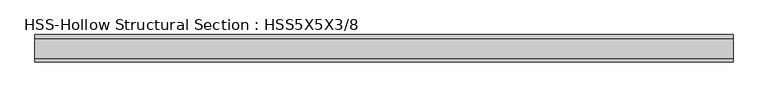
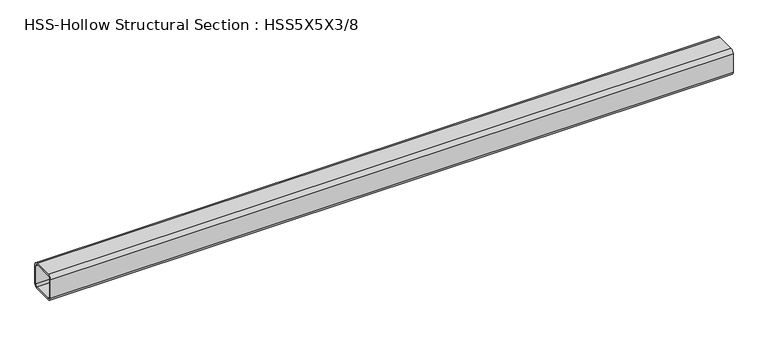
"""IFC4 building model written with IfcOpenShell, lengths in millimetres: member geometry, HSS-Hollow Structural Section : HSS5X5X3/8."""

import ifcopenshell
import ifcopenshell.guid

model = None  # the IFC model being written
_history = None  # IfcOwnerHistory: only IFC2X3 demands one
_inside = {}  # id of a spatial element -> (the spatial element, [elements in it])
_under = {}  # id of a project, library or spatial element -> (it, [spatial elements below it])
_declared = {}  # id of a project -> (the project, [libraries it declares])
_typed = {}  # id of a type object -> (the type object, [elements of that type])
_made_of = {}  # id of a material, layer set ... -> (it, [elements and type objects made of it])


def new_model(schema):
    """Start an empty IFC model of exactly this schema.

    Asked for "IFC4X3", IfcOpenShell would pick the latest addendum, in which some entities
    have other attributes; the version numbers below select the first issue.
    IFC2X3 requires an IfcOwnerHistory on every rooted entity: one is made here for all.
    """
    global model, _history
    if schema == "IFC4X3":
        model = ifcopenshell.file(schema_version=(4, 3, 0, 0))
    else:
        model = ifcopenshell.file(schema=schema)
    _inside.clear()
    _under.clear()
    _declared.clear()
    _typed.clear()
    _made_of.clear()
    _history = None
    if model.schema == "IFC2X3":
        org = make("IfcOrganization", Name="unknown")
        user = make(
            "IfcPersonAndOrganization",
            ThePerson=make("IfcPerson", FamilyName="unknown"),
            TheOrganization=org,
        )
        app = make(
            "IfcApplication",
            ApplicationDeveloper=org,
            Version="unknown",
            ApplicationFullName="unknown",
            ApplicationIdentifier="unknown",
        )
        _history = make(
            "IfcOwnerHistory",
            OwningUser=user,
            OwningApplication=app,
            ChangeAction="ADDED",
            CreationDate=0,
        )
    return model


def make(cls, **values):
    """One entity of the class cls with the attributes given. An attribute that is None is left unset."""
    return model.create_entity(
        cls, **{name: value for name, value in values.items() if value is not None}
    )


def rooted(cls, **values):
    """An entity with a GlobalId (a new one), such as an element, a storey or a relation."""
    return make(cls, GlobalId=ifcopenshell.guid.new(), OwnerHistory=_history, **values)


def si_unit(unit_type, name, prefix=None):
    """IfcSIUnit, for example si_unit("LENGTHUNIT", "METRE", prefix="MILLI")."""
    return make("IfcSIUnit", UnitType=unit_type, Prefix=prefix, Name=name)


def assignment(units):
    """IfcUnitAssignment: the units of a project."""
    return None if units is None else make("IfcUnitAssignment", Units=units)


def point(xyz):
    """IfcCartesianPoint."""
    return None if xyz is None else make("IfcCartesianPoint", Coordinates=xyz)


def direction(xyz):
    """IfcDirection."""
    return None if xyz is None else make("IfcDirection", DirectionRatios=xyz)


def frame(location, z_axis=None, x_axis=None):
    """IfcAxis2Placement3D, a coordinate frame: its origin and axes. An axis left out is left unset."""
    return make(
        "IfcAxis2Placement3D",
        Location=point(location),
        Axis=direction(z_axis),
        RefDirection=direction(x_axis),
    )


def frame_2d(location, x_axis=None):
    """IfcAxis2Placement2D, a coordinate frame in the plane: its origin and x axis."""
    return make(
        "IfcAxis2Placement2D", Location=point(location), RefDirection=direction(x_axis)
    )


def origin():
    """The frame at (0, 0, 0) with its axes left unset."""
    return frame((0.0, 0.0, 0.0))


def place(relative_to, where):
    """IfcLocalPlacement: puts the frame where relative to a parent placement (None: the world)."""
    return make(
        "IfcLocalPlacement", PlacementRelTo=relative_to, RelativePlacement=where
    )


def context(
    kind, dimensions, precision=None, world=None, true_north=None, identifier=None
):
    """IfcGeometricRepresentationContext, for example the 3D "Model" context."""
    return make(
        "IfcGeometricRepresentationContext",
        ContextIdentifier=identifier,
        ContextType=kind,
        CoordinateSpaceDimension=dimensions,
        Precision=precision,
        WorldCoordinateSystem=world,
        TrueNorth=true_north,
    )


def project(units=None, contexts=None):
    """IfcProject with its units and contexts."""
    return rooted(
        "IfcProject",
        Name="project",
        RepresentationContexts=contexts,
        UnitsInContext=assignment(units),
    )


def spatial(cls, under=None, at=None, **own):
    """A site, building, storey or space (cls), placed at a placement, below another one or the project."""
    s = rooted(cls, ObjectPlacement=at, **own)
    if under is not None:
        _under.setdefault(under.id(), (under, []))[1].append(s)
    return s


def polyline(points):
    """IfcPolyline through the points."""
    return make("IfcPolyline", Points=[point(p) for p in points])


def circle_curve(where, radius):
    """IfcCircle in the frame where."""
    return make("IfcCircle", Position=where, Radius=radius)


def trimmed(basis, trim1, trim2, sense, master):
    """IfcTrimmedCurve: the piece of a basis curve between two trims."""
    return make(
        "IfcTrimmedCurve",
        BasisCurve=basis,
        Trim1=trim1,
        Trim2=trim2,
        SenseAgreement=sense,
        MasterRepresentation=master,
    )


def segment(curve, same_sense, transition):
    """IfcCompositeCurveSegment."""
    return make(
        "IfcCompositeCurveSegment",
        Transition=transition,
        SameSense=same_sense,
        ParentCurve=curve,
    )


def composite_curve(segments, self_intersect=None):
    """IfcCompositeCurve: segments joined end to end."""
    return make("IfcCompositeCurve", Segments=segments, SelfIntersect=self_intersect)


def outline(outer, holes=None, kind="AREA"):
    """IfcArbitraryClosedProfileDef: a profile drawn as a closed curve; with holes, ...WithVoids."""
    if holes is None:
        return make("IfcArbitraryClosedProfileDef", ProfileType=kind, OuterCurve=outer)
    return make(
        "IfcArbitraryProfileDefWithVoids",
        ProfileType=kind,
        OuterCurve=outer,
        InnerCurves=holes,
    )


def extrude(swept, where, along, depth):
    """IfcExtrudedAreaSolid: the profile swept, set in the frame where, extruded along a direction by depth."""
    return make(
        "IfcExtrudedAreaSolid",
        SweptArea=swept,
        Position=where,
        ExtrudedDirection=direction(along),
        Depth=depth,
    )


def shape(context_of_items, identifier, shape_type, items):
    """IfcShapeRepresentation: the items that make up one representation, for example the "Body"."""
    return make(
        "IfcShapeRepresentation",
        ContextOfItems=context_of_items,
        RepresentationIdentifier=identifier,
        RepresentationType=shape_type,
        Items=items,
    )


def source(mapping_origin, context_of_items, identifier, shape_type, items):
    """IfcRepresentationMap: a shape defined once, which mapped items show again and again."""
    return make(
        "IfcRepresentationMap",
        MappingOrigin=mapping_origin,
        MappedRepresentation=shape(context_of_items, identifier, shape_type, items),
    )


def transform(
    local_origin,
    x_axis=None,
    y_axis=None,
    z_axis=None,
    scale=None,
    scale2=None,
    scale3=None,
    uniform=True,
):
    """IfcCartesianTransformationOperator3D, or its non-uniform kind. x_axis, y_axis, z_axis: its Axis1, 2, 3."""
    if uniform:
        return make(
            "IfcCartesianTransformationOperator3D",
            Axis1=direction(x_axis),
            Axis2=direction(y_axis),
            LocalOrigin=point(local_origin),
            Scale=scale,
            Axis3=direction(z_axis),
        )
    return make(
        "IfcCartesianTransformationOperator3DnonUniform",
        Axis1=direction(x_axis),
        Axis2=direction(y_axis),
        LocalOrigin=point(local_origin),
        Scale=scale,
        Axis3=direction(z_axis),
        Scale2=scale2,
        Scale3=scale3,
    )


def mapped(mapping_source, mapping_target):
    """IfcMappedItem: shows the shape of a source again, moved by a transform."""
    return make(
        "IfcMappedItem", MappingSource=mapping_source, MappingTarget=mapping_target
    )


def made_of(thing, what):
    """Note that an element or type object is made of a material, layer set ...; save() writes the relation."""
    if what is not None:
        _made_of.setdefault(what.id(), (what, []))[1].append(thing)
    return thing


def element(
    cls,
    number,
    at=None,
    inside=None,
    cuts=None,
    type_object=None,
    material=None,
    context=None,
    identifier="Body",
    shape_type=None,
    held_by="IfcProductDefinitionShape",
    body=None,
    shapes=None,
    **own,
):
    """One element of the class cls, such as IfcWall. Its Tag is "e" and its number.

    at: its placement. inside: the storey or other place that contains it. cuts: it is an
    opening in that element (IfcRelVoidsElement). A single representation is given by context,
    identifier, shape_type and body (its items); several are given by shapes. held_by: the class
    of the entity that holds the representations. save() writes the other relations.
    """
    e = rooted(cls, Tag="e%d" % number, ObjectPlacement=at, **own)
    if body is not None:
        shapes = [shape(context, identifier, shape_type, body)]
    if shapes is not None:
        e.Representation = make(held_by, Representations=shapes)
    if inside is not None:
        _inside.setdefault(inside.id(), (inside, []))[1].append(e)
    if cuts is not None:
        rooted(
            "IfcRelVoidsElement", RelatingBuildingElement=cuts, RelatedOpeningElement=e
        )
    if type_object is not None:
        _typed.setdefault(type_object.id(), (type_object, []))[1].append(e)
    return made_of(e, material)


def aggregate(whole, parts):
    """IfcRelAggregates: a whole, such as a stair, and the parts it consists of."""
    return rooted("IfcRelAggregates", RelatingObject=whole, RelatedObjects=parts)


def save(model, path):
    """Write the relations noted so far, then the file.

    IfcRelAggregates (storeys below a building ...), IfcRelContainedInSpatialStructure (elements
    in a storey), IfcRelDefinesByType, IfcRelAssociatesMaterial and IfcRelDeclares: one each for
    every whole, place, type object, material and project.
    """
    for whole, parts in _under.values():
        aggregate(whole, parts)
    for where, things in _inside.values():
        rooted(
            "IfcRelContainedInSpatialStructure",
            RelatedElements=things,
            RelatingStructure=where,
        )
    for kind, things in _typed.values():
        rooted("IfcRelDefinesByType", RelatedObjects=things, RelatingType=kind)
    for what, things in _made_of.values():
        rooted("IfcRelAssociatesMaterial", RelatedObjects=things, RelatingMaterial=what)
    for by, libraries in _declared.values():
        rooted("IfcRelDeclares", RelatingContext=by, RelatedDefinitions=libraries)
    model.write(path)


def hss_hollow_structural_section_hss5x5x3_8_1bfc15f5(model_context):
    return source(origin(), model_context, "Body", "SweptSolid", [
        extrude(outline(composite_curve([segment(polyline([(63.5, 45.7708), (63.5, -45.7708)]), True, "CONTINUOUS"), segment(trimmed(circle_curve(frame_2d((45.7708, -45.7708)), 17.7292), [point((63.5, -45.7708))], [point((45.7708, -63.5))], False, "CARTESIAN"), True, "CONTINUOUS"), segment(polyline([(45.7708, -63.5), (-45.7708, -63.5)]), True, "CONTINUOUS"), segment(trimmed(circle_curve(frame_2d((-45.7708, -45.7708)), 17.7292), [point((-45.7708, -63.5))], [point((-63.5, -45.7708))], False, "CARTESIAN"), True, "CONTINUOUS"), segment(polyline([(-63.5, -45.7708), (-63.5, 45.7708)]), True, "CONTINUOUS"), segment(trimmed(circle_curve(frame_2d((-45.7708, 45.7708)), 17.7292), [point((-63.5, 45.7708))], [point((-45.7708, 63.5))], False, "CARTESIAN"), True, "CONTINUOUS"), segment(polyline([(-45.7708, 63.5), (45.7708, 63.5)]), True, "CONTINUOUS"), segment(trimmed(circle_curve(frame_2d((45.7708, 45.7708)), 17.7292), [point((45.7708, 63.5))], [point((63.5, 45.7708))], False, "CARTESIAN"), True, "CONTINUOUS")], self_intersect=False), holes=[composite_curve([segment(trimmed(circle_curve(frame_2d((-45.7708, 45.7708)), 8.8646), [point((-45.7708, 54.6354))], [point((-54.6354, 45.7708))], True, "CARTESIAN"), True, "CONTINUOUS"), segment(polyline([(-54.6354, 45.7708), (-54.6354, -45.7708)]), True, "CONTINUOUS"), segment(trimmed(circle_curve(frame_2d((-45.7708, -45.7708)), 8.8646), [point((-54.6354, -45.7708))], [point((-45.7708, -54.6354))], True, "CARTESIAN"), True, "CONTINUOUS"), segment(polyline([(-45.7708, -54.6354), (45.7708, -54.6354)]), True, "CONTINUOUS"), segment(trimmed(circle_curve(frame_2d((45.7708, -45.7708)), 8.8646), [point((45.7708, -54.6354))], [point((54.6354, -45.7708))], True, "CARTESIAN"), True, "CONTINUOUS"), segment(polyline([(54.6354, -45.7708), (54.6354, 45.7708)]), True, "CONTINUOUS"), segment(trimmed(circle_curve(frame_2d((45.7708, 45.7708)), 8.8646), [point((54.6354, 45.7708))], [point((45.7708, 54.6354))], True, "CARTESIAN"), True, "CONTINUOUS"), segment(polyline([(45.7708, 54.6354), (-45.7708, 54.6354)]), True, "CONTINUOUS")], self_intersect=False)]), frame((-1559.4617293, 0.0, 0.0), z_axis=(1.0, 0.0, 0.0), x_axis=(0.0, 1.0, 0.0)), (0.0, 0.0, 1.0), 3220.1428771),
    ])


if __name__ == "__main__":
    model = new_model("IFC4")
    model_context = context("Model", 3, world=origin())
    ifc_project = project(units=[si_unit("LENGTHUNIT", "METRE", prefix="MILLI")], contexts=[model_context])
    site = spatial("IfcSite", under=ifc_project)
    building = spatial("IfcBuilding", under=site)
    placement = place(None, origin())
    hss_hollow_structural_section_hss5x5x3_8_shape = hss_hollow_structural_section_hss5x5x3_8_1bfc15f5(model_context)
    element("IfcMember", 1, ObjectType="HSS-Hollow Structural Section : HSS5X5X3/8", at=placement, inside=building, context=model_context, shape_type="MappedRepresentation", body=[
        mapped(hss_hollow_structural_section_hss5x5x3_8_shape, transform((0.0, 0.0, 0.0), x_axis=(1.0, 0.0, 0.0), y_axis=(0.0, 1.0, 0.0), z_axis=(0.0, 0.0, 1.0))),
    ])
    save(model, "model.ifc")

# Revit data of these elements
# Type "HSS-Hollow Structural Section : HSS5X5X3/8"
#   Assembly Code = "B10"
#   Shape = "Square"
#   W = 22.3
#   Ht = 0' - 5"
#   Length [instance default] = 5' - 0"
#   b = 0' - 5"
#   kr = 0' - 0.698"
#   t = 0' - 0.349"
#   A = 0.0429167 SF
#   Structural Material [instance default] = Steel ASTM A500, Grade B, Rectangular and Square
# Element 1 (IfcMember, "HSS-Hollow Structural Section : HSS5X5X3/8")
#   Materials on its faces: "Steel ASTM A500, Grade B, Rectangular and Square"
# Materials
#   "Steel ASTM A500, Grade B, Rectangular and Square": class "Metal", colour RGB 199 199 199, transparency 0, Description = "Carbon steel", Cost = 0
